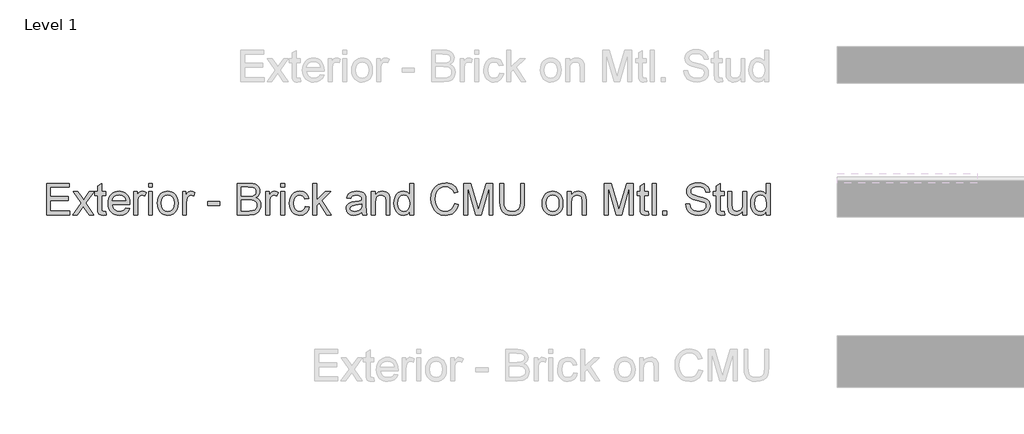
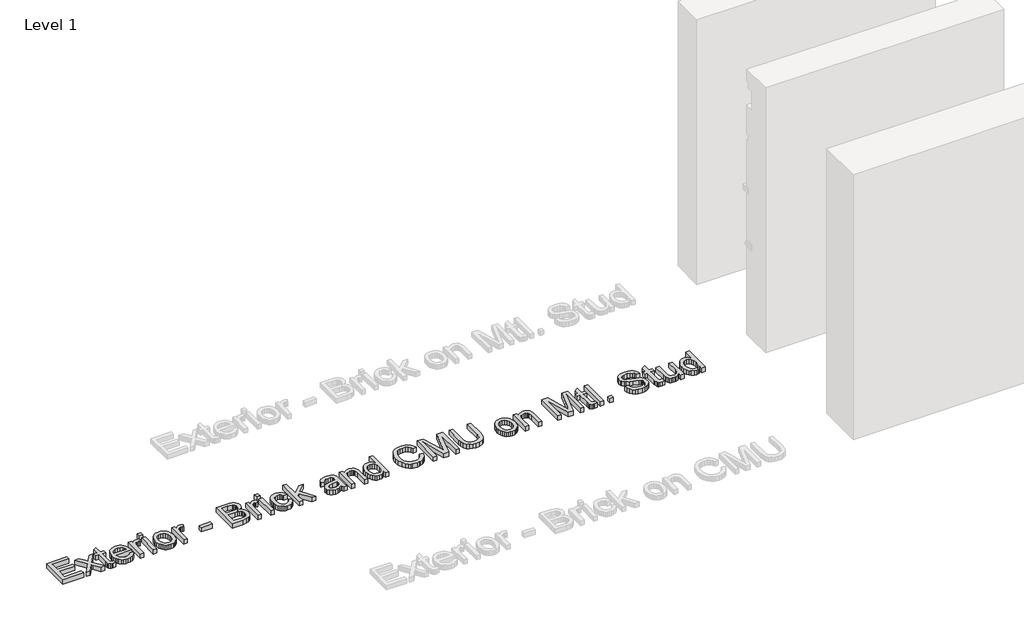
# One storey, part 26 of 42: 1 proxy.
"""IFC4 building model written with IfcOpenShell, lengths in millimetres."""

from ifc_helpers import new_model, si_unit, origin, origin_with_axes, place, context, project, spatial, polyline, outline, extrude, element, save

model = new_model("IFC4")

# Units and contexts
model_context = context("Model", 3, world=origin())
ifc_project = project(units=[si_unit("LENGTHUNIT", "METRE", prefix="MILLI")], contexts=[model_context])

# Site, building, storey
site = spatial("IfcSite", under=ifc_project)
building = spatial("IfcBuilding", under=site)
storey = spatial("IfcBuildingStorey", under=building, Name="Level 1", Elevation=0.0)

# Proxy
placement = place(None, origin())
element("IfcBuildingElementProxy", 1, Name="8\" Arial", ObjectType="8\" Arial", at=placement, inside=storey, context=model_context, shape_type="SweptSolid", body=[
    extrude(outline(polyline([(-6951.4343185, 9947.9863349), (-6951.4343185, 10252.553429), (-6732.5267197, 10252.553429), (-6732.5267197, 10214.4825422), (-6913.3634318, 10214.4825422), (-6913.3634318, 10124.0641861), (-6742.0444414, 10124.0641861), (-6742.0444414, 10085.9932994), (-6913.3634318, 10085.9932994), (-6913.3634318, 9986.0572216), (-6727.7678588, 9986.0572216), (-6727.7678588, 9947.9863349), (-6951.4343185, 9947.9863349)])), origin_with_axes(), (0.0, 0.0, 1.0), 50.8),
    extrude(outline(polyline([(-6699.2146938, 9947.9863349), (-6617.8679162, 10060.4144223), (-6694.4558329, 10171.6527946), (-6648.6517973, 10171.6527946), (-6611.6962685, 10118.1156101), (-6594.445398, 10092.8341619), (-6579.4996006, 10113.5054636), (-6537.413425, 10171.6527946), (-6491.6093894, 10171.6527946), (-6572.0638806, 10060.4144223), (-6494.5836774, 9947.9863349), (-6540.3877131, 9947.9863349), (-6587.0096779, 10015.5770303), (-6595.560756, 10027.9203256), (-6653.4106581, 9947.9863349), (-6699.2146938, 9947.9863349)])), origin_with_axes(), (0.0, 0.0, 1.0), 50.8),
    extrude(outline(polyline([(-6380.3710172, 9979.7368596), (-6375.6121563, 9946.8709769), (-6404.0909642, 9943.227474), (-6422.3642463, 9944.8075646), (-6435.9902033, 9949.5478361), (-6445.6194608, 9956.8534311), (-6451.9026442, 9966.1294919), (-6455.3602541, 9982.0605221), (-6456.5127907, 10009.3310255), (-6456.5127907, 10133.5819078), (-6485.0659557, 10133.5819078), (-6485.0659557, 10171.6527946), (-6456.5127907, 10171.6527946), (-6456.5127907, 10226.0079083), (-6418.4419039, 10248.3894257), (-6418.4419039, 10171.6527946), (-6380.3710172, 10171.6527946), (-6380.3710172, 10133.5819078), (-6418.4419039, 10133.5819078), (-6418.4419039, 10010.4463835), (-6416.4342595, 9990.8160825), (-6409.9280044, 9983.8636842), (-6396.9526729, 9981.2983608), (-6380.3710172, 9979.7368596)])), origin_with_axes(), (0.0, 0.0, 1.0), 50.8),
    extrude(outline(polyline([(-6185.7038657, 10014.6103867), (-6148.376551, 10009.8515259), (-6161.8259096, 9981.7259147), (-6183.2872567, 9960.7014162), (-6212.2772703, 9947.5959596), (-6248.3126287, 9943.227474), (-6271.9349819, 9945.1119643), (-6292.982717, 9950.7654353), (-6311.4558341, 9960.1878868), (-6327.3543331, 9973.3793189), (-6340.1391243, 9989.972593), (-6349.271118, 10009.6005703), (-6354.7503142, 10032.2632509), (-6356.5767129, 10057.9606347), (-6354.7317249, 10084.529392), (-6349.1967608, 10107.9472629), (-6339.9718205, 10128.2142474), (-6327.0569043, 10145.3303455), (-6311.2002312, 10158.9284186), (-6293.1500207, 10168.641328), (-6272.9062728, 10174.4690736), (-6250.4689875, 10176.4116554), (-6228.7543613, 10174.4737209), (-6209.1170893, 10168.6599173), (-6191.5571716, 10158.9702446), (-6176.0746082, 10145.4047027), (-6163.4362078, 10128.3257832), (-6154.4087789, 10108.0959773), (-6148.9923215, 10084.715285), (-6147.1868358, 10058.1837063), (-6147.4099074, 10047.9224126), (-6318.5058262, 10047.9224126), (-6311.9159193, 10019.4250155), (-6296.6076306, 9998.4748742), (-6274.5142473, 9985.5924891), (-6247.5690567, 9981.2983608), (-6227.3067195, 9983.2874159), (-6210.241742, 9989.2545813), (-6196.374124, 9999.5716429), (-6185.7038657, 10014.6103867)]), holes=[polyline([(-6318.5058262, 10085.9932994), (-6185.2577225, 10085.9932994), (-6190.4069587, 10106.1069222), (-6200.5009487, 10120.4950405), (-6222.6965731, 10133.8793366), (-6250.6177019, 10138.3407687), (-6276.2802308, 10134.7809177), (-6297.499917, 10124.1013647), (-6312.2505267, 10107.4546464), (-6318.5058262, 10085.9932994)])]), origin_with_axes(), (0.0, 0.0, 1.0), 50.8),
    extrude(outline(polyline([(-6109.115949, 9947.9863349), (-6109.115949, 10171.6527946), (-6075.8039231, 10171.6527946), (-6075.8039231, 10138.5638403), (-6063.4978064, 10157.7479981), (-6052.1583333, 10169.0502926), (-6040.7816816, 10174.5713147), (-6028.364029, 10176.4116554), (-6009.4029429, 10173.474546), (-5990.1444279, 10164.6632177), (-6002.8595092, 10130.5332626), (-6016.2438053, 10136.3888922), (-6029.6281015, 10138.3407687), (-6040.9954585, 10136.4632494), (-6051.1545111, 10130.8306914), (-6059.3616871, 10121.8706487), (-6064.8734146, 10110.0106752), (-6069.5021503, 10088.7445158), (-6071.0450622, 10065.5450692), (-6071.0450622, 9947.9863349), (-6109.115949, 9947.9863349)])), origin_with_axes(), (0.0, 0.0, 1.0), 50.8),
    extrude(outline(polyline([(-5966.3501237, 10214.4825422), (-5966.3501237, 10252.553429), (-5928.2792369, 10252.553429), (-5928.2792369, 10214.4825422), (-5966.3501237, 10214.4825422)])), origin_with_axes(), (0.0, 0.0, 1.0), 50.8),
    extrude(outline(polyline([(-5966.3501237, 9947.9863349), (-5966.3501237, 10171.6527946), (-5928.2792369, 10171.6527946), (-5928.2792369, 9947.9863349), (-5966.3501237, 9947.9863349)])), origin_with_axes(), (0.0, 0.0, 1.0), 50.8),
    extrude(outline(polyline([(-5880.6906284, 10059.8195647), (-5878.6318635, 10088.7863417), (-5872.4555685, 10113.7471245), (-5862.1617435, 10134.7019132), (-5847.7503885, 10151.6507076), (-5833.2414398, 10162.4836223), (-5817.2267577, 10170.2214185), (-5799.7063422, 10174.8640962), (-5780.6801935, 10176.4116554), (-5759.676608, 10174.5271651), (-5740.6853142, 10168.8736942), (-5723.7063121, 10159.4512427), (-5708.7396018, 10146.2598106), (-5696.524108, 10129.745541), (-5687.7987552, 10110.3545773), (-5682.5635435, 10088.0869193), (-5680.818473, 10062.9425672), (-5683.9042968, 10024.4813051), (-5693.1617683, 9995.2031573), (-5708.3213426, 9973.2770778), (-5729.1134748, 9956.8720204), (-5753.8093601, 9946.6386106), (-5780.6801935, 9943.227474), (-5801.9905025, 9945.1049934), (-5821.1583946, 9950.7375513), (-5838.1838699, 9960.1251479), (-5853.0669284, 9973.2677831), (-5865.1522972, 9989.9423854), (-5873.7847034, 10009.9258831), (-5878.9641472, 10033.2182762), (-5880.6906284, 10059.8195647)]), holes=[polyline([(-5842.6197417, 10059.8939219), (-5838.2140775, 10025.4386541), (-5824.9970851, 10000.8914832), (-5805.1065339, 9986.1966414), (-5780.6801935, 9981.2983608), (-5756.3653889, 9986.2245253), (-5736.5120163, 10001.003019), (-5723.2950239, 10025.8755026), (-5718.8893597, 10061.0836372), (-5723.3229078, 10094.5350828), (-5736.6235521, 10118.7476463), (-5756.5048086, 10133.4424881), (-5780.6801935, 10138.3407687), (-5805.1065339, 10133.4610774), (-5824.9970851, 10118.8220035), (-5838.2140775, 10094.3306005), (-5842.6197417, 10059.8939219)])]), origin_with_axes(), (0.0, 0.0, 1.0), 50.8),
    extrude(outline(polyline([(-5637.9887254, 9947.9863349), (-5637.9887254, 10171.6527946), (-5604.6766995, 10171.6527946), (-5604.6766995, 10138.5638403), (-5592.3705827, 10157.7479981), (-5581.0311096, 10169.0502926), (-5569.6544579, 10174.5713147), (-5557.2368054, 10176.4116554), (-5538.2757192, 10173.474546), (-5519.0172042, 10164.6632177), (-5531.7322856, 10130.5332626), (-5545.1165817, 10136.3888922), (-5558.5008778, 10138.3407687), (-5569.8682349, 10136.4632494), (-5580.0272874, 10130.8306914), (-5588.2344634, 10121.8706487), (-5593.7461909, 10110.0106752), (-5598.3749267, 10088.7445158), (-5599.9178386, 10065.5450692), (-5599.9178386, 9947.9863349), (-5637.9887254, 9947.9863349)])), origin_with_axes(), (0.0, 0.0, 1.0), 50.8),
    extrude(outline(polyline([(-5395.2868223, 10038.4046909), (-5395.2868223, 10076.4755777), (-5276.3153012, 10076.4755777), (-5276.3153012, 10038.4046909), (-5395.2868223, 10038.4046909)])), origin_with_axes(), (0.0, 0.0, 1.0), 50.8),
    extrude(outline(polyline([(-5109.7551716, 9947.9863349), (-5109.7551716, 10252.553429), (-4993.5348669, 10252.553429), (-4961.5705652, 10250.3134183), (-4936.6144298, 10243.5933863), (-4917.4860399, 10232.2260292), (-4903.004975, 10216.0440434), (-4893.8869233, 10197.0086), (-4890.8475727, 10177.0808702), (-4893.4036015, 10158.7425256), (-4901.0716878, 10141.5009497), (-4913.9075996, 10126.4157326), (-4931.9671047, 10114.5464645), (-4910.3942219, 10103.2813486), (-4894.453897, 10086.1420138), (-4884.6108625, 10064.2624075), (-4881.329851, 10038.7764769), (-4883.5698617, 10017.5382015), (-4890.2898937, 9997.842838), (-4900.3188212, 9981.0938785), (-4912.4855181, 9968.6948153), (-4927.3848422, 9959.7161833), (-4945.611651, 9953.2285175), (-4994.4271533, 9947.9863349), (-5109.7551716, 9947.9863349)]), holes=[polyline([(-5071.6842848, 10128.823047), (-5002.1603022, 10128.823047), (-4961.5612706, 10132.0947638), (-4947.3497506, 10137.7366164), (-4937.1349302, 10146.1854534), (-4930.9725772, 10157.3111495), (-4928.9184595, 10170.9835798), (-4930.8331574, 10184.2563401), (-4936.5772512, 10195.8188848), (-4945.8904905, 10204.8439901), (-4958.5126254, 10210.504432), (-5007.4396634, 10214.4825422), (-5071.6842848, 10214.4825422), (-5071.6842848, 10128.823047)]), polyline([(-5071.6842848, 9986.0572216), (-4993.6092241, 9986.0572216), (-4965.3534878, 9987.5443657), (-4941.4476478, 9995.8351935), (-4925.6095641, 10012.7514567), (-4920.9529444, 10024.7043767), (-4919.4007378, 10038.4046909), (-4921.2224892, 10054.3171319), (-4926.6877435, 10067.9988568), (-4936.2333491, 10078.6969991), (-4950.2961547, 10085.658692), (-4970.2145898, 10089.4787932), (-4997.3270841, 10090.7521602), (-5071.6842848, 10090.7521602), (-5071.6842848, 9986.0572216)])]), origin_with_axes(), (0.0, 0.0, 1.0), 50.8),
    extrude(outline(polyline([(-4833.7412426, 9947.9863349), (-4833.7412426, 10171.6527946), (-4800.4292167, 10171.6527946), (-4800.4292167, 10138.5638403), (-4788.1231, 10157.7479981), (-4776.7836269, 10169.0502926), (-4765.4069751, 10174.5713147), (-4752.9893226, 10176.4116554), (-4734.0282365, 10173.474546), (-4714.7697215, 10164.6632177), (-4727.4848028, 10130.5332626), (-4740.8690989, 10136.3888922), (-4754.253395, 10138.3407687), (-4765.6207521, 10136.4632494), (-4775.7798046, 10130.8306914), (-4783.9869807, 10121.8706487), (-4789.4987082, 10110.0106752), (-4794.1274439, 10088.7445158), (-4795.6703558, 10065.5450692), (-4795.6703558, 9947.9863349), (-4833.7412426, 9947.9863349)])), origin_with_axes(), (0.0, 0.0, 1.0), 50.8),
    extrude(outline(polyline([(-4690.9754172, 9947.9863349), (-4690.9754172, 10171.6527946), (-4652.9045305, 10171.6527946), (-4652.9045305, 9947.9863349), (-4690.9754172, 9947.9863349)])), origin_with_axes(), (0.0, 0.0, 1.0), 50.8),
    extrude(outline(polyline([(-4690.9754172, 10214.4825422), (-4690.9754172, 10252.553429), (-4652.9045305, 10252.553429), (-4652.9045305, 10214.4825422), (-4690.9754172, 10214.4825422)])), origin_with_axes(), (0.0, 0.0, 1.0), 50.8),
    extrude(outline(polyline([(-4453.032375, 10028.8869693), (-4414.9614882, 10024.1281084), (-4425.5759786, 9990.2676981), (-4445.5222977, 9964.6795264), (-4472.9229262, 9948.5904871), (-4505.9003447, 9943.227474), (-4527.2524796, 9945.0980224), (-4546.3971351, 9950.7096674), (-4563.3343113, 9960.062409), (-4578.064008, 9973.1562473), (-4589.9867204, 9989.7448741), (-4598.5029435, 10009.581981), (-4603.6126774, 10032.6675682), (-4605.315922, 10059.0016355), (-4602.4066966, 10092.8806351), (-4593.6790201, 10122.2424347), (-4578.993473, 10145.9530871), (-4558.2106354, 10162.8786449), (-4533.3474464, 10173.0284028), (-4506.4208451, 10176.4116554), (-4474.2520612, 10171.7643304), (-4448.5337644, 10157.8223553), (-4430.0838839, 10135.3293021), (-4419.7203491, 10105.0287428), (-4457.7912358, 10100.2698819), (-4464.6971609, 10116.8794216), (-4475.451071, 10128.7858684), (-4489.4581087, 10135.9520436), (-4506.1234163, 10138.3407687), (-4530.7263551, 10133.6376757), (-4550.2544149, 10119.5283969), (-4562.9973802, 10095.2507709), (-4567.2450353, 10060.0426363), (-4563.0903267, 10024.3604747), (-4550.6262009, 9999.9991968), (-4531.4513378, 9985.9735698), (-4507.1644171, 9981.2983608), (-4487.4504643, 9984.2168809), (-4471.2870678, 9992.9724413), (-4459.5293354, 10007.7881136), (-4453.032375, 10028.8869693)])), origin_with_axes(), (0.0, 0.0, 1.0), 50.8),
    extrude(outline(polyline([(-4381.6494623, 9947.9863349), (-4381.6494623, 10252.553429), (-4343.5785756, 10252.553429), (-4343.5785756, 10088.8932302), (-4258.2165092, 10171.6527946), (-4205.5716111, 10171.6527946), (-4291.9746783, 10087.8522294), (-4200.8127502, 9947.9863349), (-4245.2783562, 9947.9863349), (-4319.2637709, 10061.381066), (-4343.5785756, 10037.8098333), (-4343.5785756, 9947.9863349), (-4381.6494623, 9947.9863349)])), origin_with_axes(), (0.0, 0.0, 1.0), 50.8),
    extrude(outline(polyline([(-3905.7633779, 9976.5395), (-3923.9530081, 9960.9430771), (-3942.681728, 9950.7375513), (-3962.3770915, 9945.1049934), (-3983.4666526, 9943.227474), (-4015.2822398, 9947.744674), (-4038.7512313, 9961.2962738), (-4053.2230015, 9981.8746291), (-4058.0469249, 10007.4720954), (-4056.2251735, 10023.2544113), (-4050.7599192, 10037.5867617), (-4042.3296716, 10049.8556998), (-4031.61294, 10059.4477787), (-4004.9558836, 10071.9397885), (-3972.0156437, 10077.6652929), (-3933.0896491, 10083.6882262), (-3905.9864495, 10090.7521602), (-3905.7633779, 10099.2288811), (-3908.3844692, 10116.2195015), (-3916.2477431, 10127.335903), (-3933.8332211, 10135.5895523), (-3958.3339187, 10138.3407687), (-3981.012865, 10136.5097226), (-3996.8509487, 10131.0165844), (-4007.6513321, 10120.8575319), (-4015.2171773, 10105.0287428), (-4053.288064, 10109.7876036), (-4046.6795678, 10130.6076198), (-4036.8179441, 10146.966204), (-4022.7830225, 10159.476803), (-4003.6546326, 10168.7528638), (-3980.2599983, 10174.4969575), (-3953.4263435, 10176.4116554), (-3927.6894574, 10174.7200291), (-3907.2877005, 10169.6451502), (-3891.9050546, 10162.0142425), (-3881.2255016, 10152.6545298), (-3874.1429783, 10141.0826905), (-3869.5514211, 10126.8154026), (-3867.6924911, 10093.5033767), (-3867.6924911, 10046.1378398), (-3865.7592039, 9979.9971098), (-3858.1747694, 9947.9863349), (-3896.2456562, 9947.9863349), (-3902.3429466, 9961.2219166), (-3905.7633779, 9976.5395)]), holes=[polyline([(-3905.7633779, 10052.6812735), (-3967.1824256, 10041.007193), (-3999.9367725, 10034.8355453), (-4014.7710341, 10024.7973232), (-4019.9760381, 10010.1489547), (-4017.1411698, 9998.8280709), (-4008.636565, 9989.5520101), (-3994.6481166, 9983.3617731), (-3975.3617177, 9981.2983608), (-3954.9134875, 9983.5755501), (-3936.8446877, 9990.4071179), (-3922.1963192, 10000.4732239), (-3912.0093827, 10012.4540279), (-3907.4921828, 10024.7973232), (-3905.9864495, 10041.8994794), (-3905.7633779, 10052.6812735)])]), origin_with_axes(), (0.0, 0.0, 1.0), 50.8),
    extrude(outline(polyline([(-3815.3450218, 9947.9863349), (-3815.3450218, 10171.6527946), (-3777.274135, 10171.6527946), (-3777.274135, 10140.4227703), (-3764.047848, 10156.1679075), (-3748.163291, 10167.4144342), (-3729.620464, 10174.1623501), (-3708.4193672, 10176.4116554), (-3689.6534687, 10174.5991987), (-3672.4676607, 10169.1618284), (-3658.1353102, 10160.778054), (-3647.9297844, 10150.126385), (-3636.5159541, 10122.1308989), (-3634.5083097, 10085.3240846), (-3634.5083097, 9947.9863349), (-3672.5791965, 9947.9863349), (-3672.5791965, 10080.1934377), (-3676.9662713, 10113.8772497), (-3683.0356778, 10123.9061771), (-3692.4697476, 10131.6857992), (-3704.5620874, 10136.6770263), (-3718.6063037, 10138.3407687), (-3740.9041692, 10134.6043193), (-3759.9117287, 10123.3949713), (-3767.5077815, 10114.2443883), (-3772.9335334, 10101.7384366), (-3777.274135, 10066.6604272), (-3777.274135, 9947.9863349), (-3815.3450218, 9947.9863349)])), origin_with_axes(), (0.0, 0.0, 1.0), 50.8),
    extrude(outline(polyline([(-3444.1538759, 9947.9863349), (-3444.1538759, 9983.9008628), (-3455.5444696, 9966.1062552), (-3469.3423776, 9953.3958212), (-3485.5476001, 9945.7695608), (-3504.1601369, 9943.227474), (-3528.7723703, 9946.9081555), (-3551.3026021, 9957.9501998), (-3570.3752241, 9975.582151), (-3584.614628, 9999.0325532), (-3593.4817242, 10027.353352), (-3596.4374229, 10059.5964931), (-3593.7140905, 10091.4399643), (-3585.544093, 10120.1976117), (-3571.9367253, 10144.2335768), (-3552.9012819, 10161.9120013), (-3529.8784337, 10172.7867419), (-3504.3088513, 10176.4116554), (-3485.6823725, 10173.8184481), (-3469.2122525, 10166.0388259), (-3455.2516881, 10154.1137899), (-3444.1538759, 10139.0843407), (-3444.1538759, 10252.553429), (-3406.0829891, 10252.553429), (-3406.0829891, 9947.9863349), (-3444.1538759, 9947.9863349)]), holes=[polyline([(-3558.3665362, 10059.7452075), (-3554.0724078, 10025.308529), (-3541.1900228, 10000.817126), (-3522.4705975, 9986.1780521), (-3500.6653484, 9981.2983608), (-3478.869394, 9985.9549805), (-3460.6239959, 9999.9248396), (-3448.2714059, 10023.4681882), (-3444.1538759, 10056.8452767), (-3448.3457631, 10093.336073), (-3460.9214247, 10118.6361105), (-3479.6315553, 10133.4146041), (-3502.2268496, 10138.3407687), (-3524.2551704, 10133.6097918), (-3542.3053808, 10119.4168611), (-3554.3512473, 10095.0369939), (-3558.3665362, 10059.7452075)])]), origin_with_axes(), (0.0, 0.0, 1.0), 50.8),
    extrude(outline(polyline([(-3011.097539, 10056.2504191), (-2973.0266523, 10046.4352686), (-2980.5599662, 10022.7594712), (-2990.5935409, 10002.0719037), (-3003.1273766, 9984.3725663), (-3018.1614731, 9969.6614589), (-3035.3565758, 9958.0965905), (-3054.3734298, 9949.8359703), (-3075.2120353, 9944.8795981), (-3097.8723922, 9943.227474), (-3142.0312748, 9948.2279958), (-3160.7019032, 9954.478648), (-3177.0999896, 9963.229561), (-3203.9801176, 9987.7116694), (-3223.57324, 10021.1538204), (-3235.5354547, 10060.4701902), (-3239.5228596, 10102.5749551), (-3235.0149543, 10146.9847933), (-3221.4912384, 10185.3345195), (-3199.6581054, 10216.4065348), (-3170.2219485, 10238.9832398), (-3135.3112428, 10252.7300273), (-3097.054463, 10257.3122898), (-3075.2794215, 10255.8297931), (-3055.3121895, 10251.382303), (-3037.1527669, 10243.9698196), (-3020.8011537, 10233.5923428), (-3006.5268948, 10220.5240648), (-2994.5995351, 10205.0391777), (-2977.7855131, 10166.8195765), (-3015.8563999, 10157.7479981), (-3029.054803, 10185.5111179), (-3047.0864242, 10204.5558559), (-3070.174335, 10215.5700163), (-3098.541607, 10219.241403), (-3131.2401861, 10215.1703463), (-3158.1017248, 10202.9571761), (-3178.4848925, 10183.8845541), (-3191.7483581, 10159.2351421), (-3199.0260691, 10131.3697811), (-3201.4519728, 10102.6493123), (-3198.5799259, 10067.4783564), (-3189.9637853, 10037.0662613), (-3175.2782382, 10012.5748583), (-3154.1979718, 9995.1659787), (-3128.9258182, 9984.7652653), (-3101.6646095, 9981.2983608), (-3069.8862008, 9986.020043), (-3043.4057427, 10000.1850898), (-3023.4129504, 10023.6447866), (-3011.097539, 10056.2504191)])), origin_with_axes(), (0.0, 0.0, 1.0), 50.8),
    extrude(outline(polyline([(-2920.679183, 9947.9863349), (-2920.679183, 10252.553429), (-2855.1704892, 10252.553429), (-2792.859155, 10037.8841905), (-2780.2927881, 9993.0467985), (-2766.6854203, 10041.6020506), (-2705.4150869, 10252.553429), (-2639.9063931, 10252.553429), (-2639.9063931, 9947.9863349), (-2677.9772799, 9947.9863349), (-2677.9772799, 10214.4825422), (-2754.4908394, 9947.9863349), (-2806.0947367, 9947.9863349), (-2882.6082962, 10214.4825422), (-2882.6082962, 9947.9863349), (-2920.679183, 9947.9863349)])), origin_with_axes(), (0.0, 0.0, 1.0), 50.8),
    extrude(outline(polyline([(-2373.4101858, 10252.553429), (-2335.3392991, 10252.553429), (-2335.3392991, 10076.8473637), (-2337.9232118, 10035.6999478), (-2345.67495, 10004.0144856), (-2360.1560148, 9979.5695559), (-2382.9279075, 9960.1437372), (-2414.046396, 9947.4565398), (-2453.5672482, 9943.227474), (-2492.2236979, 9946.9081555), (-2523.1284094, 9957.9501998), (-2546.2906774, 9975.9725263), (-2561.7197966, 10000.5940544), (-2570.3917051, 10033.6179461), (-2573.2823413, 10076.8473637), (-2573.2823413, 10252.553429), (-2535.2114545, 10252.553429), (-2535.2114545, 10078.1857933), (-2533.3339352, 10043.9721863), (-2527.7013773, 10020.1499982), (-2517.4958515, 10003.6519943), (-2501.8994286, 9991.4109401), (-2481.5627342, 9983.8265056), (-2457.1363938, 9981.2983608), (-2418.4148815, 9986.2988825), (-2403.9198747, 9992.5495347), (-2392.6687008, 10001.3004478), (-2384.2431005, 10013.6065645), (-2378.2248146, 10030.5228277), (-2373.4101858, 10078.1857933), (-2373.4101858, 10252.553429)])), origin_with_axes(), (0.0, 0.0, 1.0), 50.8),
    extrude(outline(polyline([(-2164.0203086, 10059.8195647), (-2161.9615437, 10088.7863417), (-2155.7852487, 10113.7471245), (-2145.4914237, 10134.7019132), (-2131.0800687, 10151.6507076), (-2116.57112, 10162.4836223), (-2100.5564378, 10170.2214185), (-2083.0360224, 10174.8640962), (-2064.0098737, 10176.4116554), (-2043.0062882, 10174.5271651), (-2024.0149944, 10168.8736942), (-2007.0359923, 10159.4512427), (-1992.069282, 10146.2598106), (-1979.8537882, 10129.745541), (-1971.1284354, 10110.3545773), (-1965.8932237, 10088.0869193), (-1964.1481532, 10062.9425672), (-1967.233977, 10024.4813051), (-1976.4914485, 9995.2031573), (-1991.6510228, 9973.2770778), (-2012.443155, 9956.8720204), (-2037.1390403, 9946.6386106), (-2064.0098737, 9943.227474), (-2085.3201827, 9945.1049934), (-2104.4880748, 9950.7375513), (-2121.5135501, 9960.1251479), (-2136.3966086, 9973.2677831), (-2148.4819774, 9989.9423854), (-2157.1143836, 10009.9258831), (-2162.2938274, 10033.2182762), (-2164.0203086, 10059.8195647)]), holes=[polyline([(-2125.9494219, 10059.8939219), (-2121.5437577, 10025.4386541), (-2108.3267653, 10000.8914832), (-2088.4362141, 9986.1966414), (-2064.0098737, 9981.2983608), (-2039.6950691, 9986.2245253), (-2019.8416965, 10001.003019), (-2006.6247041, 10025.8755026), (-2002.2190399, 10061.0836372), (-2006.652588, 10094.5350828), (-2019.9532323, 10118.7476463), (-2039.8344888, 10133.4424881), (-2064.0098737, 10138.3407687), (-2088.4362141, 10133.4610774), (-2108.3267653, 10118.8220035), (-2121.5437577, 10094.3306005), (-2125.9494219, 10059.8939219)])]), origin_with_axes(), (0.0, 0.0, 1.0), 50.8),
    extrude(outline(polyline([(-1921.3184056, 9947.9863349), (-1921.3184056, 10171.6527946), (-1883.2475188, 10171.6527946), (-1883.2475188, 10140.4227703), (-1870.0212317, 10156.1679075), (-1854.1366747, 10167.4144342), (-1835.5938478, 10174.1623501), (-1814.392751, 10176.4116554), (-1795.6268524, 10174.5991987), (-1778.4410444, 10169.1618284), (-1764.108694, 10160.778054), (-1753.9031682, 10150.126385), (-1742.4893379, 10122.1308989), (-1740.4816935, 10085.3240846), (-1740.4816935, 9947.9863349), (-1778.5525802, 9947.9863349), (-1778.5525802, 10080.1934377), (-1782.9396551, 10113.8772497), (-1789.0090616, 10123.9061771), (-1798.4431314, 10131.6857992), (-1810.5354712, 10136.6770263), (-1824.5796875, 10138.3407687), (-1846.877553, 10134.6043193), (-1865.8851124, 10123.3949713), (-1873.4811652, 10114.2443883), (-1878.9069172, 10101.7384366), (-1883.2475188, 10066.6604272), (-1883.2475188, 9947.9863349), (-1921.3184056, 9947.9863349)])), origin_with_axes(), (0.0, 0.0, 1.0), 50.8),
    extrude(outline(polyline([(-1564.4038422, 9947.9863349), (-1564.4038422, 10252.553429), (-1498.8951484, 10252.553429), (-1436.5838142, 10037.8841905), (-1424.0174473, 9993.0467985), (-1410.4100795, 10041.6020506), (-1349.1397462, 10252.553429), (-1283.6310524, 10252.553429), (-1283.6310524, 9947.9863349), (-1321.7019391, 9947.9863349), (-1321.7019391, 10214.4825422), (-1398.2154986, 9947.9863349), (-1449.8193959, 9947.9863349), (-1526.3329554, 10214.4825422), (-1526.3329554, 9947.9863349), (-1564.4038422, 9947.9863349)])), origin_with_axes(), (0.0, 0.0, 1.0), 50.8),
    extrude(outline(polyline([(-1140.865227, 9979.7368596), (-1136.1063662, 9946.8709769), (-1164.585174, 9943.227474), (-1182.8584561, 9944.8075646), (-1196.4844131, 9949.5478361), (-1206.1136706, 9956.8534311), (-1212.3968541, 9966.1294919), (-1215.8544639, 9982.0605221), (-1217.0070005, 10009.3310255), (-1217.0070005, 10133.5819078), (-1245.5601656, 10133.5819078), (-1245.5601656, 10171.6527946), (-1217.0070005, 10171.6527946), (-1217.0070005, 10226.0079083), (-1178.9361138, 10248.3894257), (-1178.9361138, 10171.6527946), (-1140.865227, 10171.6527946), (-1140.865227, 10133.5819078), (-1178.9361138, 10133.5819078), (-1178.9361138, 10010.4463835), (-1176.9284694, 9990.8160825), (-1170.4222143, 9983.8636842), (-1157.4468828, 9981.2983608), (-1140.865227, 9979.7368596)])), origin_with_axes(), (0.0, 0.0, 1.0), 50.8),
    extrude(outline(polyline([(-1102.7943403, 9947.9863349), (-1102.7943403, 10252.553429), (-1064.7234535, 10252.553429), (-1064.7234535, 9947.9863349), (-1102.7943403, 9947.9863349)])), origin_with_axes(), (0.0, 0.0, 1.0), 50.8),
    extrude(outline(polyline([(-998.0994017, 9947.9863349), (-998.0994017, 9986.0572216), (-960.0285149, 9986.0572216), (-960.0285149, 9947.9863349), (-998.0994017, 9947.9863349)])), origin_with_axes(), (0.0, 0.0, 1.0), 50.8),
    extrude(outline(polyline([(-779.1918028, 10052.6812735), (-741.120916, 10052.6812735), (-736.7524305, 10031.5545338), (-728.8519779, 10014.5732081), (-716.5272719, 10001.0959655), (-698.886026, 9990.4814751), (-677.3224378, 9983.5941394), (-653.2307048, 9981.2983608), (-632.0203133, 9983.0364604), (-613.4496024, 9988.2507591), (-598.401564, 9996.5044083), (-587.7591896, 10007.3605596), (-581.4295329, 10019.8246854), (-579.3196473, 10032.9022581), (-580.8997378, 10045.6452234), (-585.6400094, 10056.6593837), (-595.2692669, 10066.056275), (-611.5163152, 10073.9474329), (-666.9496083, 10088.4842656), (-703.3381634, 10098.1042285), (-726.6212619, 10107.2594588), (-745.5730534, 10120.0674866), (-759.0038228, 10135.5895523), (-767.0065165, 10153.4910483), (-769.6740811, 10173.4373674), (-766.3744803, 10195.735233), (-756.475678, 10216.5273652), (-740.2379243, 10234.1500218), (-717.9214694, 10246.9394603), (-691.1342879, 10254.7190824), (-661.4843541, 10257.3122898), (-629.3620434, 10254.598252), (-601.2550215, 10246.4561385), (-578.1671107, 10233.0532531), (-561.1021332, 10214.5568994), (-550.3017497, 10192.1196141), (-546.0076214, 10166.8939338), (-584.0785082, 10166.8939338), (-591.068085, 10189.6100586), (-605.6420964, 10206.0058213), (-628.4139891, 10215.9325076), (-659.9972101, 10219.241403), (-692.3240031, 10215.9696862), (-714.5010382, 10206.1545357), (-727.3276553, 10191.7106495), (-731.6031944, 10174.5527254), (-728.5731384, 10159.9229462), (-719.4829706, 10148.1559192), (-697.9937396, 10137.6343753), (-657.3203509, 10126.8897598), (-615.3457111, 10116.684234), (-589.952727, 10107.7799592), (-568.2497191, 10093.9681092), (-553.1087341, 10076.9217209), (-544.2137539, 10056.8266874), (-541.2487606, 10033.8689017), (-544.6598971, 10010.3999102), (-554.8933069, 9988.3251163), (-571.5307305, 9969.3268515), (-594.1539089, 9955.0874476), (-621.3593497, 9946.1924674), (-651.7435608, 9943.227474), (-689.0429916, 9946.4248337), (-719.7432208, 9956.0169126), (-744.1974452, 9972.0408893), (-762.7588615, 9994.5339425), (-774.6746029, 10021.934571), (-779.1918028, 10052.6812735)])), origin_with_axes(), (0.0, 0.0, 1.0), 50.8),
    extrude(outline(polyline([(-408.0006569, 9979.7368596), (-403.2417961, 9946.8709769), (-431.7206039, 9943.227474), (-449.993886, 9944.8075646), (-463.619843, 9949.5478361), (-473.2491005, 9956.8534311), (-479.532284, 9966.1294919), (-482.9898938, 9982.0605221), (-484.1424304, 10009.3310255), (-484.1424304, 10133.5819078), (-512.6955955, 10133.5819078), (-512.6955955, 10171.6527946), (-484.1424304, 10171.6527946), (-484.1424304, 10226.0079083), (-446.0715437, 10248.3894257), (-446.0715437, 10171.6527946), (-408.0006569, 10171.6527946), (-408.0006569, 10133.5819078), (-446.0715437, 10133.5819078), (-446.0715437, 10010.4463835), (-444.0638992, 9990.8160825), (-437.5576442, 9983.8636842), (-424.5823127, 9981.2983608), (-408.0006569, 9979.7368596)])), origin_with_axes(), (0.0, 0.0, 1.0), 50.8),
    extrude(outline(polyline([(-227.1639448, 9947.9863349), (-227.1639448, 9986.4290077), (-240.9386162, 9967.5283367), (-256.9811823, 9954.0278574), (-275.291643, 9945.9275699), (-295.8699983, 9943.227474), (-314.4128252, 9945.1235827), (-331.6729904, 9950.8119085), (-346.1540552, 9959.3629866), (-356.359581, 9969.8473519), (-363.2283274, 9982.5810225), (-367.6990541, 9997.8800166), (-369.9297702, 10033.2740441), (-369.9297702, 10171.6527946), (-331.8588834, 10171.6527946), (-331.8588834, 10051.1941295), (-329.5538102, 10012.3796707), (-324.0049041, 9999.4322231), (-314.496477, 9989.5891887), (-301.6605653, 9983.3710678), (-286.129205, 9981.2983608), (-269.7055583, 9983.417541), (-254.3415017, 9989.7750817), (-241.6728936, 9999.7854198), (-233.3355925, 10012.8629925), (-228.7068567, 10030.7737832), (-227.1639448, 10055.2837755), (-227.1639448, 10171.6527946), (-189.093058, 10171.6527946), (-189.093058, 9947.9863349), (-227.1639448, 9947.9863349)])), origin_with_axes(), (0.0, 0.0, 1.0), 50.8),
    extrude(outline(polyline([(1.2613757, 9947.9863349), (1.2613757, 9983.9008628), (-10.1292179, 9966.1062552), (-23.927126, 9953.3958212), (-40.1323484, 9945.7695608), (-58.7448852, 9943.227474), (-83.3571187, 9946.9081555), (-105.8873505, 9957.9501998), (-124.9599724, 9975.582151), (-139.1993764, 9999.0325532), (-148.0664726, 10027.353352), (-151.0221713, 10059.5964931), (-148.2988388, 10091.4399643), (-140.1288414, 10120.1976117), (-126.5214737, 10144.2335768), (-107.4860303, 10161.9120013), (-84.463182, 10172.7867419), (-58.8935996, 10176.4116554), (-40.2671208, 10173.8184481), (-23.7970009, 10166.0388259), (-9.8364365, 10154.1137899), (1.2613757, 10139.0843407), (1.2613757, 10252.553429), (39.3322625, 10252.553429), (39.3322625, 9947.9863349), (1.2613757, 9947.9863349)]), holes=[polyline([(-112.9512845, 10059.7452075), (-108.6571562, 10025.308529), (-95.7747712, 10000.817126), (-77.0553459, 9986.1780521), (-55.2500968, 9981.2983608), (-33.4541423, 9985.9549805), (-15.2087442, 9999.9248396), (-2.8561542, 10023.4681882), (1.2613757, 10056.8452767), (-2.9305114, 10093.336073), (-15.506173, 10118.6361105), (-34.2163036, 10133.4146041), (-56.811598, 10138.3407687), (-78.8399187, 10133.6097918), (-96.8901292, 10119.4168611), (-108.9359957, 10095.0369939), (-112.9512845, 10059.7452075)])]), origin_with_axes(), (0.0, 0.0, 1.0), 50.8),
])

save(model, "model.ifc")

# Revit data of these elements
# Element 1 (IfcBuildingElementProxy, "8\" Arial")
#   Phase Created = New Construction
